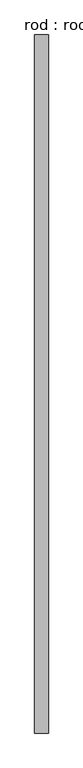
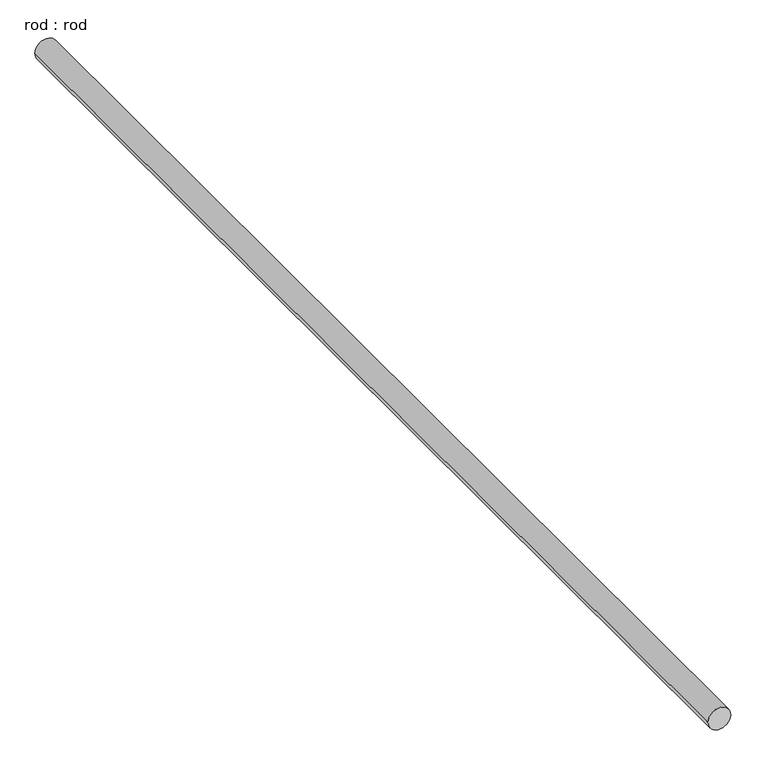
"""IFC4 building model written with IfcOpenShell, lengths in millimetres: proxy geometry, rod : rod."""

import ifcopenshell
import ifcopenshell.guid

model = None  # the IFC model being written
_history = None  # IfcOwnerHistory: only IFC2X3 demands one
_inside = {}  # id of a spatial element -> (the spatial element, [elements in it])
_under = {}  # id of a project, library or spatial element -> (it, [spatial elements below it])
_declared = {}  # id of a project -> (the project, [libraries it declares])
_typed = {}  # id of a type object -> (the type object, [elements of that type])
_made_of = {}  # id of a material, layer set ... -> (it, [elements and type objects made of it])


def new_model(schema):
    """Start an empty IFC model of exactly this schema.

    Asked for "IFC4X3", IfcOpenShell would pick the latest addendum, in which some entities
    have other attributes; the version numbers below select the first issue.
    IFC2X3 requires an IfcOwnerHistory on every rooted entity: one is made here for all.
    """
    global model, _history
    if schema == "IFC4X3":
        model = ifcopenshell.file(schema_version=(4, 3, 0, 0))
    else:
        model = ifcopenshell.file(schema=schema)
    _inside.clear()
    _under.clear()
    _declared.clear()
    _typed.clear()
    _made_of.clear()
    _history = None
    if model.schema == "IFC2X3":
        org = make("IfcOrganization", Name="unknown")
        user = make(
            "IfcPersonAndOrganization",
            ThePerson=make("IfcPerson", FamilyName="unknown"),
            TheOrganization=org,
        )
        app = make(
            "IfcApplication",
            ApplicationDeveloper=org,
            Version="unknown",
            ApplicationFullName="unknown",
            ApplicationIdentifier="unknown",
        )
        _history = make(
            "IfcOwnerHistory",
            OwningUser=user,
            OwningApplication=app,
            ChangeAction="ADDED",
            CreationDate=0,
        )
    return model


def make(cls, **values):
    """One entity of the class cls with the attributes given. An attribute that is None is left unset."""
    return model.create_entity(
        cls, **{name: value for name, value in values.items() if value is not None}
    )


def rooted(cls, **values):
    """An entity with a GlobalId (a new one), such as an element, a storey or a relation."""
    return make(cls, GlobalId=ifcopenshell.guid.new(), OwnerHistory=_history, **values)


def si_unit(unit_type, name, prefix=None):
    """IfcSIUnit, for example si_unit("LENGTHUNIT", "METRE", prefix="MILLI")."""
    return make("IfcSIUnit", UnitType=unit_type, Prefix=prefix, Name=name)


def assignment(units):
    """IfcUnitAssignment: the units of a project."""
    return None if units is None else make("IfcUnitAssignment", Units=units)


def point(xyz):
    """IfcCartesianPoint."""
    return None if xyz is None else make("IfcCartesianPoint", Coordinates=xyz)


def direction(xyz):
    """IfcDirection."""
    return None if xyz is None else make("IfcDirection", DirectionRatios=xyz)


def frame(location, z_axis=None, x_axis=None):
    """IfcAxis2Placement3D, a coordinate frame: its origin and axes. An axis left out is left unset."""
    return make(
        "IfcAxis2Placement3D",
        Location=point(location),
        Axis=direction(z_axis),
        RefDirection=direction(x_axis),
    )


def frame_2d(location, x_axis=None):
    """IfcAxis2Placement2D, a coordinate frame in the plane: its origin and x axis."""
    return make(
        "IfcAxis2Placement2D", Location=point(location), RefDirection=direction(x_axis)
    )


def origin():
    """The frame at (0, 0, 0) with its axes left unset."""
    return frame((0.0, 0.0, 0.0))


def place(relative_to, where):
    """IfcLocalPlacement: puts the frame where relative to a parent placement (None: the world)."""
    return make(
        "IfcLocalPlacement", PlacementRelTo=relative_to, RelativePlacement=where
    )


def context(
    kind, dimensions, precision=None, world=None, true_north=None, identifier=None
):
    """IfcGeometricRepresentationContext, for example the 3D "Model" context."""
    return make(
        "IfcGeometricRepresentationContext",
        ContextIdentifier=identifier,
        ContextType=kind,
        CoordinateSpaceDimension=dimensions,
        Precision=precision,
        WorldCoordinateSystem=world,
        TrueNorth=true_north,
    )


def project(units=None, contexts=None):
    """IfcProject with its units and contexts."""
    return rooted(
        "IfcProject",
        Name="project",
        RepresentationContexts=contexts,
        UnitsInContext=assignment(units),
    )


def spatial(cls, under=None, at=None, **own):
    """A site, building, storey or space (cls), placed at a placement, below another one or the project."""
    s = rooted(cls, ObjectPlacement=at, **own)
    if under is not None:
        _under.setdefault(under.id(), (under, []))[1].append(s)
    return s


def circle_curve(where, radius):
    """IfcCircle in the frame where."""
    return make("IfcCircle", Position=where, Radius=radius)


def trimmed(basis, trim1, trim2, sense, master):
    """IfcTrimmedCurve: the piece of a basis curve between two trims."""
    return make(
        "IfcTrimmedCurve",
        BasisCurve=basis,
        Trim1=trim1,
        Trim2=trim2,
        SenseAgreement=sense,
        MasterRepresentation=master,
    )


def segment(curve, same_sense, transition):
    """IfcCompositeCurveSegment."""
    return make(
        "IfcCompositeCurveSegment",
        Transition=transition,
        SameSense=same_sense,
        ParentCurve=curve,
    )


def composite_curve(segments, self_intersect=None):
    """IfcCompositeCurve: segments joined end to end."""
    return make("IfcCompositeCurve", Segments=segments, SelfIntersect=self_intersect)


def outline(outer, holes=None, kind="AREA"):
    """IfcArbitraryClosedProfileDef: a profile drawn as a closed curve; with holes, ...WithVoids."""
    if holes is None:
        return make("IfcArbitraryClosedProfileDef", ProfileType=kind, OuterCurve=outer)
    return make(
        "IfcArbitraryProfileDefWithVoids",
        ProfileType=kind,
        OuterCurve=outer,
        InnerCurves=holes,
    )


def extrude(swept, where, along, depth):
    """IfcExtrudedAreaSolid: the profile swept, set in the frame where, extruded along a direction by depth."""
    return make(
        "IfcExtrudedAreaSolid",
        SweptArea=swept,
        Position=where,
        ExtrudedDirection=direction(along),
        Depth=depth,
    )


def shape(context_of_items, identifier, shape_type, items):
    """IfcShapeRepresentation: the items that make up one representation, for example the "Body"."""
    return make(
        "IfcShapeRepresentation",
        ContextOfItems=context_of_items,
        RepresentationIdentifier=identifier,
        RepresentationType=shape_type,
        Items=items,
    )


def source(mapping_origin, context_of_items, identifier, shape_type, items):
    """IfcRepresentationMap: a shape defined once, which mapped items show again and again."""
    return make(
        "IfcRepresentationMap",
        MappingOrigin=mapping_origin,
        MappedRepresentation=shape(context_of_items, identifier, shape_type, items),
    )


def transform(
    local_origin,
    x_axis=None,
    y_axis=None,
    z_axis=None,
    scale=None,
    scale2=None,
    scale3=None,
    uniform=True,
):
    """IfcCartesianTransformationOperator3D, or its non-uniform kind. x_axis, y_axis, z_axis: its Axis1, 2, 3."""
    if uniform:
        return make(
            "IfcCartesianTransformationOperator3D",
            Axis1=direction(x_axis),
            Axis2=direction(y_axis),
            LocalOrigin=point(local_origin),
            Scale=scale,
            Axis3=direction(z_axis),
        )
    return make(
        "IfcCartesianTransformationOperator3DnonUniform",
        Axis1=direction(x_axis),
        Axis2=direction(y_axis),
        LocalOrigin=point(local_origin),
        Scale=scale,
        Axis3=direction(z_axis),
        Scale2=scale2,
        Scale3=scale3,
    )


def mapped(mapping_source, mapping_target):
    """IfcMappedItem: shows the shape of a source again, moved by a transform."""
    return make(
        "IfcMappedItem", MappingSource=mapping_source, MappingTarget=mapping_target
    )


def made_of(thing, what):
    """Note that an element or type object is made of a material, layer set ...; save() writes the relation."""
    if what is not None:
        _made_of.setdefault(what.id(), (what, []))[1].append(thing)
    return thing


def element(
    cls,
    number,
    at=None,
    inside=None,
    cuts=None,
    type_object=None,
    material=None,
    context=None,
    identifier="Body",
    shape_type=None,
    held_by="IfcProductDefinitionShape",
    body=None,
    shapes=None,
    **own,
):
    """One element of the class cls, such as IfcWall. Its Tag is "e" and its number.

    at: its placement. inside: the storey or other place that contains it. cuts: it is an
    opening in that element (IfcRelVoidsElement). A single representation is given by context,
    identifier, shape_type and body (its items); several are given by shapes. held_by: the class
    of the entity that holds the representations. save() writes the other relations.
    """
    e = rooted(cls, Tag="e%d" % number, ObjectPlacement=at, **own)
    if body is not None:
        shapes = [shape(context, identifier, shape_type, body)]
    if shapes is not None:
        e.Representation = make(held_by, Representations=shapes)
    if inside is not None:
        _inside.setdefault(inside.id(), (inside, []))[1].append(e)
    if cuts is not None:
        rooted(
            "IfcRelVoidsElement", RelatingBuildingElement=cuts, RelatedOpeningElement=e
        )
    if type_object is not None:
        _typed.setdefault(type_object.id(), (type_object, []))[1].append(e)
    return made_of(e, material)


def aggregate(whole, parts):
    """IfcRelAggregates: a whole, such as a stair, and the parts it consists of."""
    return rooted("IfcRelAggregates", RelatingObject=whole, RelatedObjects=parts)


def save(model, path):
    """Write the relations noted so far, then the file.

    IfcRelAggregates (storeys below a building ...), IfcRelContainedInSpatialStructure (elements
    in a storey), IfcRelDefinesByType, IfcRelAssociatesMaterial and IfcRelDeclares: one each for
    every whole, place, type object, material and project.
    """
    for whole, parts in _under.values():
        aggregate(whole, parts)
    for where, things in _inside.values():
        rooted(
            "IfcRelContainedInSpatialStructure",
            RelatedElements=things,
            RelatingStructure=where,
        )
    for kind, things in _typed.values():
        rooted("IfcRelDefinesByType", RelatedObjects=things, RelatingType=kind)
    for what, things in _made_of.values():
        rooted("IfcRelAssociatesMaterial", RelatedObjects=things, RelatingMaterial=what)
    for by, libraries in _declared.values():
        rooted("IfcRelDeclares", RelatingContext=by, RelatedDefinitions=libraries)
    model.write(path)


def rod_rod_9264356c(model_context):
    return source(origin(), model_context, "Body", "SweptSolid", [
        extrude(outline(composite_curve([segment(trimmed(circle_curve(frame_2d((0.0108462, 0.0)), 200.0), [point((0.0108462, 200.0))], [point((0.0108462, -200.0))], False, "CARTESIAN"), True, "CONTINUOUS"), segment(trimmed(circle_curve(frame_2d((0.0108462, 0.0)), 200.0), [point((0.0108462, -200.0))], [point((0.0108462, 200.0))], False, "CARTESIAN"), True, "CONTINUOUS")], self_intersect=False)), frame((0.0, -6136.6802752, 0.0), z_axis=(0.0, 1.0, 0.0), x_axis=(0.0, 0.0, 1.0)), (0.0, 0.0, 1.0), 20458.8177811),
    ])


if __name__ == "__main__":
    model = new_model("IFC4")
    model_context = context("Model", 3, world=origin())
    ifc_project = project(units=[si_unit("LENGTHUNIT", "METRE", prefix="MILLI")], contexts=[model_context])
    site = spatial("IfcSite", under=ifc_project)
    building = spatial("IfcBuilding", under=site)
    placement = place(None, origin())
    rod_rod_shape = rod_rod_9264356c(model_context)
    element("IfcBuildingElementProxy", 1, Name="rod : rod", ObjectType="rod : rod", at=placement, inside=building, context=model_context, shape_type="MappedRepresentation", body=[
        mapped(rod_rod_shape, transform((0.0, 0.0, 0.0), x_axis=(1.0, 0.0, 0.0), y_axis=(0.0, 1.0, 0.0), z_axis=(0.0, 0.0, 1.0))),
    ])
    save(model, "model.ifc")

# Revit data of these elements
# Type "rod : rod"
#   Default Elevation = 0
